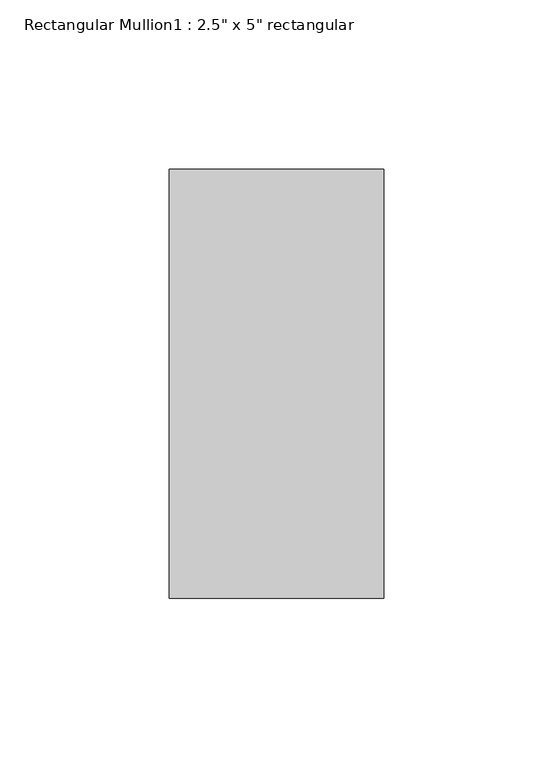
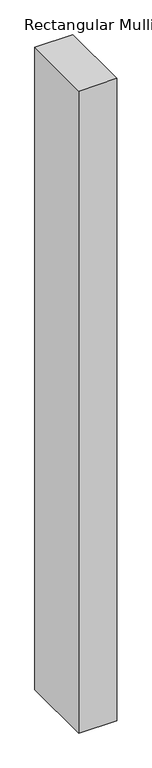
"""IFC4 building model written with IfcOpenShell, lengths in millimetres: member geometry."""

from ifc_helpers import new_model, si_unit, frame, origin, place, context, project, spatial, polyline, outline, extrude, source, transform, mapped, element, save


def member_b037884b(model_context):
    return source(origin(), model_context, "Body", "SweptSolid", [
        extrude(outline(polyline([(0.0, 63.5), (0.0, -63.5), (-63.5, -63.5), (-63.5, 63.5), (0.0, 63.5)])), frame((0.0, 0.0, -1134.5333334), z_axis=(0.0, 0.0, 1.0), x_axis=(1.0, 0.0, 0.0)), (0.0, 0.0, 1.0), 1134.5333334),
    ])


if __name__ == "__main__":
    model = new_model("IFC4")
    model_context = context("Model", 3, world=origin())
    ifc_project = project(units=[si_unit("LENGTHUNIT", "METRE", prefix="MILLI")], contexts=[model_context])
    site = spatial("IfcSite", under=ifc_project)
    building = spatial("IfcBuilding", under=site)
    placement = place(None, origin())
    member_shape = member_b037884b(model_context)
    element("IfcMember", 1, ObjectType="Rectangular Mullion1 : 2.5\" x 5\" rectangular", at=placement, inside=building, context=model_context, shape_type="MappedRepresentation", body=[
        mapped(member_shape, transform((0.0, 0.0, 0.0), x_axis=(1.0, 0.0, 0.0), y_axis=(0.0, 1.0, 0.0), z_axis=(0.0, 0.0, 1.0))),
    ])
    save(model, "model.ifc")

# Revit data of these elements
# Type "Rectangular Mullion1 : 2.5\" x 5\" rectangular"
#   built-in parameter 1007304 = 0.416667 (stored number, unit not read)
#   built-in parameter 1007301 = 0.104167 (stored number, unit not read)
#   built-in parameter 1007300 = 0.104167 (stored number, unit not read)
# Element 1 (IfcMember, "Rectangular Mullion1 : 2.5\" x 5\" rectangular")
#   Materials on its faces: "support-frame"
# Materials
#   "support-frame": class "Unassigned", colour RGB 233 233 233, transparency 0, Cost = 0
